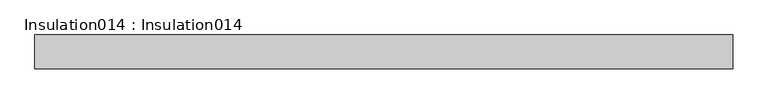
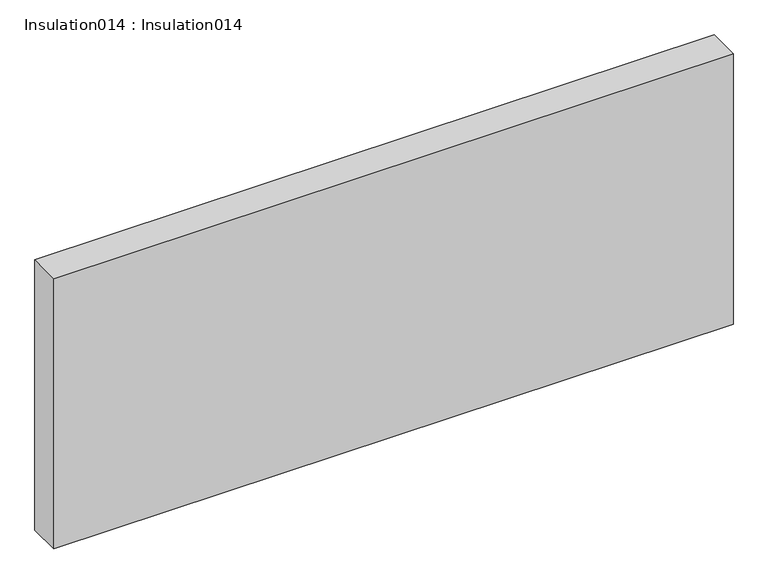
"""IFC4 building model written with IfcOpenShell, lengths in millimetres: proxy geometry, Insulation014 : Insulation014."""

from ifc_helpers import new_model, si_unit, frame, origin, place, context, project, spatial, polyline, outline, extrude, source, transform, mapped, element, save


def insulation014_insulation014_cc25b819(model_context):
    return source(origin(), model_context, "Body", "SweptSolid", [
        extrude(outline(polyline([(14382.5, -4279.1775), (14382.5, -4375.74), (12382.5, -4375.74), (12382.5, -4279.1775), (14382.5, -4279.1775)])), frame((0.0, 0.0, 40163.5), z_axis=(0.0, 0.0, 1.0), x_axis=(1.0, 0.0, 0.0)), (0.0, 0.0, 1.0), 841.3787187),
    ])


if __name__ == "__main__":
    model = new_model("IFC4")
    model_context = context("Model", 3, world=origin())
    ifc_project = project(units=[si_unit("LENGTHUNIT", "METRE", prefix="MILLI")], contexts=[model_context])
    site = spatial("IfcSite", under=ifc_project)
    building = spatial("IfcBuilding", under=site)
    placement = place(None, origin())
    insulation014_insulation014_shape = insulation014_insulation014_cc25b819(model_context)
    element("IfcBuildingElementProxy", 1, Name="Insulation014 : Insulation014", ObjectType="Insulation014 : Insulation014", at=placement, inside=building, context=model_context, shape_type="MappedRepresentation", body=[
        mapped(insulation014_insulation014_shape, transform((0.0, 0.0, 0.0), x_axis=(1.0, 0.0, 0.0), y_axis=(0.0, 1.0, 0.0), z_axis=(0.0, 0.0, 1.0))),
    ])
    save(model, "model.ifc")

# Revit data of these elements
# Type "Insulation014 : Insulation014"
#   NameOverride = "Insulation014"
# Element 1 (IfcBuildingElementProxy, "Insulation014 : Insulation014")
#   Materials on its faces: "BATT INSULATION (U-FACTOR = 0.065 MIN.) OVER CLASS II VAPOR RETARDER (TOWARDS INTERIOR)"
# Materials
#   "BATT INSULATION (U-FACTOR = 0.065 MIN.) OVER CLASS II VAPOR RETARDER (TOWARDS INTERIOR)": class "Unassigned", colour RGB 246 242 160, transparency 0, Cost = 0
